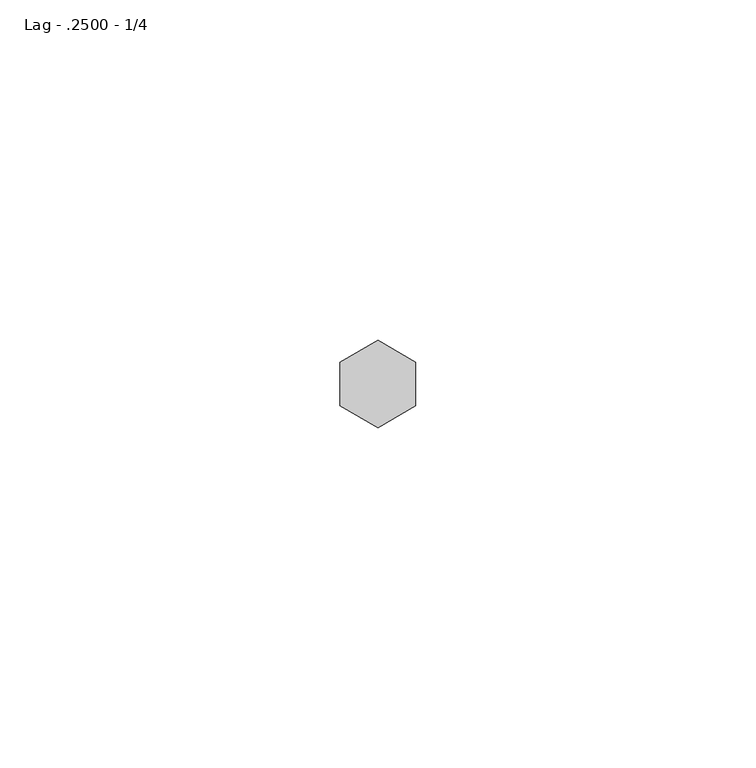
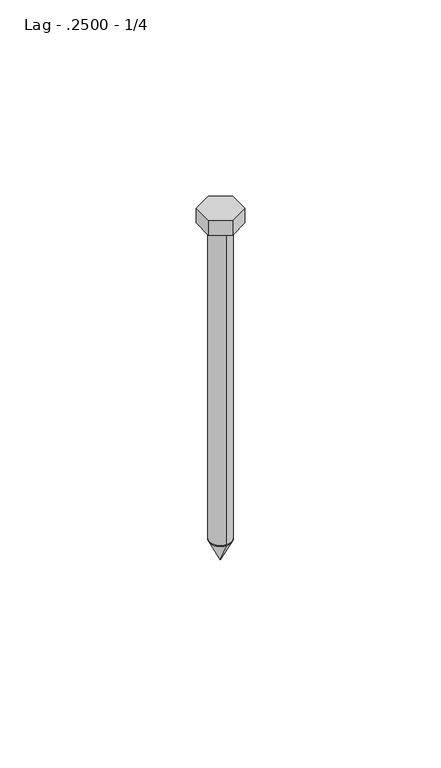
"""IFC4 building model written with IfcOpenShell, lengths in millimetres: fastener geometry, 060523 - W_P_C - Fastenings - Generic : Lag - .2500 - 1/4."""

from ifc_helpers import new_model, si_unit, point, frame, origin, origin_with_axes, origin_2d, place, context, project, spatial, polyline, circle_curve, trimmed, segment, composite_curve, outline, extrude, source, transform, mapped, element, save
from ifc_brep_helpers import plane_surface, revolved_surface, advanced_brep


def lag_2500_1_4_c9adf12f(model_context):
    return source(origin(), model_context, "Body", "SolidModel", [
        advanced_brep(
        [(0.0, -3.302, -101.6), (0.0, 3.302, -101.6), (0.0, 0.0, -101.6), (0.0, 0.0, -108.204)],
        [
            (0, 1, circle_curve(frame((0.0, 0.0, -101.6), z_axis=(0.0, 0.0, 1.0), x_axis=(0.0, 1.0, 0.0)), 3.302)),
            (1, 2),
            (2, 0),
            (1, 0, circle_curve(frame((0.0, 0.0, -101.6), z_axis=(0.0, 0.0, 1.0), x_axis=(0.0, 1.0, 0.0)), 3.302)),
            (3, 1),
            (0, 3),
        ],
        [
            plane_surface(frame((0.0, 0.0, -101.6), z_axis=(0.0, 0.0, 1.0), x_axis=(0.0, 1.0, 0.0))),
            revolved_surface(polyline([(0.0, 3.302, -101.6), (0.0, 0.0, -108.204)]), (0.0, 0.0, -103.0840259), (0.0, 0.0, -1.0)),
        ],
        [
            (0, [[1, 2, 3]]),
            (0, [[4, -3, -2]]),
            (1, [[5, -1, 6]]),
            (1, [[-6, -4, -5]]),
        ],
    ),
        extrude(outline(polyline([(-5.55625, 3.2079024), (0.0, 6.4158049), (5.55625, 3.2079024), (5.55625, -3.2079024), (0.0, -6.4158049), (-5.55625, -3.2079024), (-5.55625, 3.2079024)])), origin_with_axes(), (0.0, 0.0, 1.0), 4.7625),
        extrude(outline(composite_curve([segment(trimmed(circle_curve(origin_2d(), 3.302), [point((0.0, -3.302))], [point((0.0, 3.302))], False, "CARTESIAN"), True, "CONTINUOUS"), segment(trimmed(circle_curve(origin_2d(), 3.302), [point((0.0, 3.302))], [point((0.0, -3.302))], False, "CARTESIAN"), True, "CONTINUOUS")], self_intersect=False)), frame((0.0, 0.0, -101.6), z_axis=(0.0, 0.0, 1.0), x_axis=(1.0, 0.0, 0.0)), (0.0, 0.0, 1.0), 101.6),
    ])


if __name__ == "__main__":
    model = new_model("IFC4")
    model_context = context("Model", 3, world=origin())
    ifc_project = project(units=[si_unit("LENGTHUNIT", "METRE", prefix="MILLI")], contexts=[model_context])
    site = spatial("IfcSite", under=ifc_project)
    building = spatial("IfcBuilding", under=site)
    placement = place(None, origin())
    lag_2500_1_4_shape = lag_2500_1_4_c9adf12f(model_context)
    element("IfcFastener", 1, ObjectType="060523 - W_P_C - Fastenings - Generic : Lag - .2500 - 1/4", at=placement, inside=building, context=model_context, shape_type="MappedRepresentation", body=[
        mapped(lag_2500_1_4_shape, transform((0.0, 0.0, 0.0), x_axis=(1.0, 0.0, 0.0), y_axis=(0.0, 1.0, 0.0), z_axis=(0.0, 0.0, 1.0))),
    ])
    save(model, "model.ifc")

# Revit data of these elements
# Type "060523 - W_P_C - Fastenings - Generic : Lag - .2500 - 1/4"
#   Washer_Thickness = 0' - 0 1/16"
#   Washer Radius = 0' - 0.3175"
#   Washer Offset - Head = 0' - 0"
#   Washer Offset = 0' - 0"
#   Thickness_of_Substrate [instance default] = 0' - 1"
#   Side = 0' - 0.25293"
#   Radius = 0' - 0.13"
#   Length [instance default] = 0' - 4"
#   Head Size = 0' - 0 7/16"
#   Head Radius = 0' - 0 7/32"
#   Head Height = 0' - 0 3/16"
#   Double Diameter = 0' - 0.52"
#   Diameter = 0' - 0.26"
#   Default Elevation = 4' - 0"
#   Washer_Nut_Visibility = no
#   Washer_Head_Visibility = no
#   Round_Head_Visibility = no
#   Point Visibility = yes
#   Nut_Visibility = no
#   Hex_Head_Visiblilty = yes
#   Washer Material = none
#   Bolt Material (Size) = AT SILL - FASTENER AT 24" O.C.
# Element 1 (IfcFastener, "060523 - W_P_C - Fastenings - Generic : Lag - .2500 - 1/4")
#   Materials on its faces: "AT SILL - FASTENER AT 24\" O.C."
# Materials
#   "AT SILL - FASTENER AT 24\" O.C.": class "Generic", colour RGB 120 120 120, transparency 0, Cost = 0
